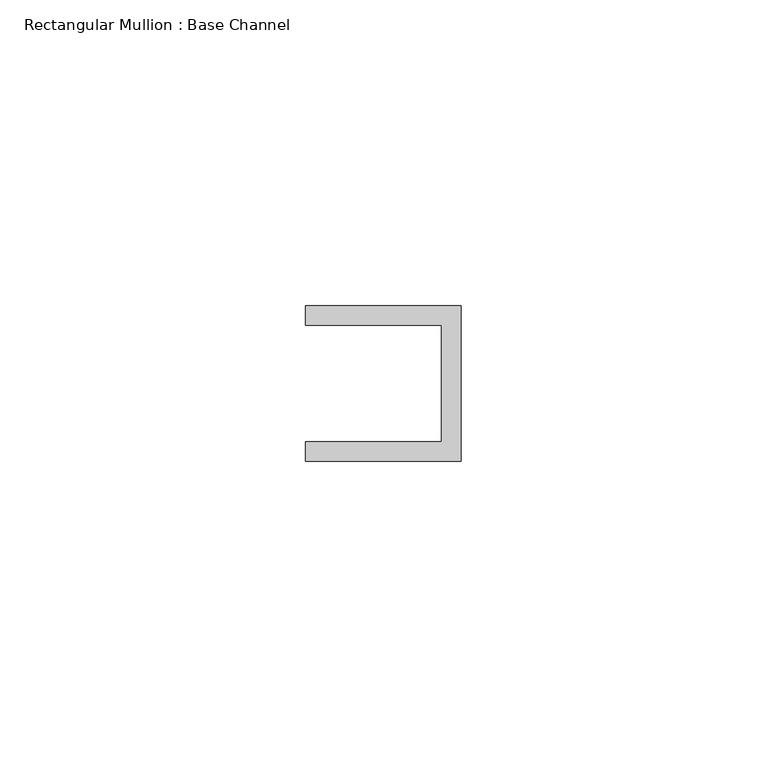
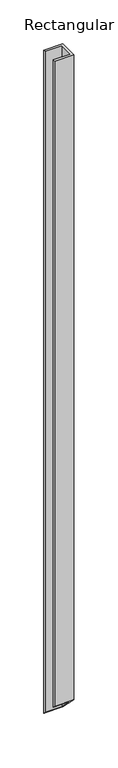
"""IFC4 building model written with IfcOpenShell, lengths in millimetres: member geometry, Rectangular Mullion : Base Channel."""

from ifc_helpers import new_model, si_unit, origin, place, context, project, spatial, faceted_brep, source, transform, mapped, element, save


def rectangular_mullion_base_channel_704ed750(model_context):
    return source(origin(), model_context, "Body", "Brep", [
        faceted_brep([(0.0, -12.7, 0.0), (0.0, 12.7, 0.0), (-25.4, 12.7, 0.0), (-25.4, 9.525, 0.0), (-3.175, 9.525, 0.0), (-3.175, -9.525, 0.0), (-25.4, -9.525, 0.0), (-25.4, -12.7, 0.0), (0.0, -12.7, -901.7000002), (0.0, 12.7, -927.1000002), (-25.4, 12.7, -927.1000002), (-25.4, 9.525, -923.9250002), (-3.175, 9.525, -923.9250002), (-3.175, -9.525, -904.8750002), (-25.4, -9.525, -904.8750002), (-25.4, -12.7, -901.7000002)], [[[0, 1, 2, 3, 4, 5, 6, 7]], [[1, 0, 8, 9]], [[2, 1, 9, 10]], [[3, 2, 10, 11]], [[4, 3, 11, 12]], [[5, 4, 12, 13]], [[6, 5, 13, 14]], [[7, 6, 14, 15]], [[0, 7, 15, 8]], [[8, 15, 14, 13, 12, 11, 10, 9]]]),
    ])


if __name__ == "__main__":
    model = new_model("IFC4")
    model_context = context("Model", 3, world=origin())
    ifc_project = project(units=[si_unit("LENGTHUNIT", "METRE", prefix="MILLI")], contexts=[model_context])
    site = spatial("IfcSite", under=ifc_project)
    building = spatial("IfcBuilding", under=site)
    placement = place(None, origin())
    rectangular_mullion_base_channel_shape = rectangular_mullion_base_channel_704ed750(model_context)
    element("IfcMember", 1, ObjectType="Rectangular Mullion : Base Channel", at=placement, inside=building, context=model_context, shape_type="MappedRepresentation", body=[
        mapped(rectangular_mullion_base_channel_shape, transform((0.0, 0.0, 0.0), x_axis=(1.0, 0.0, 0.0), y_axis=(0.0, 1.0, 0.0), z_axis=(0.0, 0.0, 1.0))),
    ])
    save(model, "model.ifc")

# Revit data of these elements
# Type "Rectangular Mullion : Base Channel"
#   built-in parameter 1007322 = 0.0833333 (stored number, unit not read)
#   built-in parameter 1007321 = 0.0416667 (stored number, unit not read)
#   built-in parameter 1007320 = -0.03125 (stored number, unit not read)
# Element 1 (IfcMember, "Rectangular Mullion : Base Channel")
#   Materials on its faces: "ALUM"
# Materials
#   "ALUM": class "Generic", colour RGB 157 157 157, transparency 0, Cost = 0
